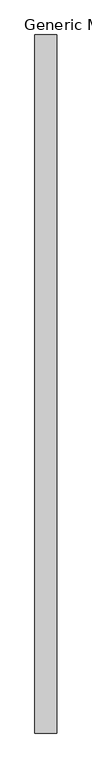
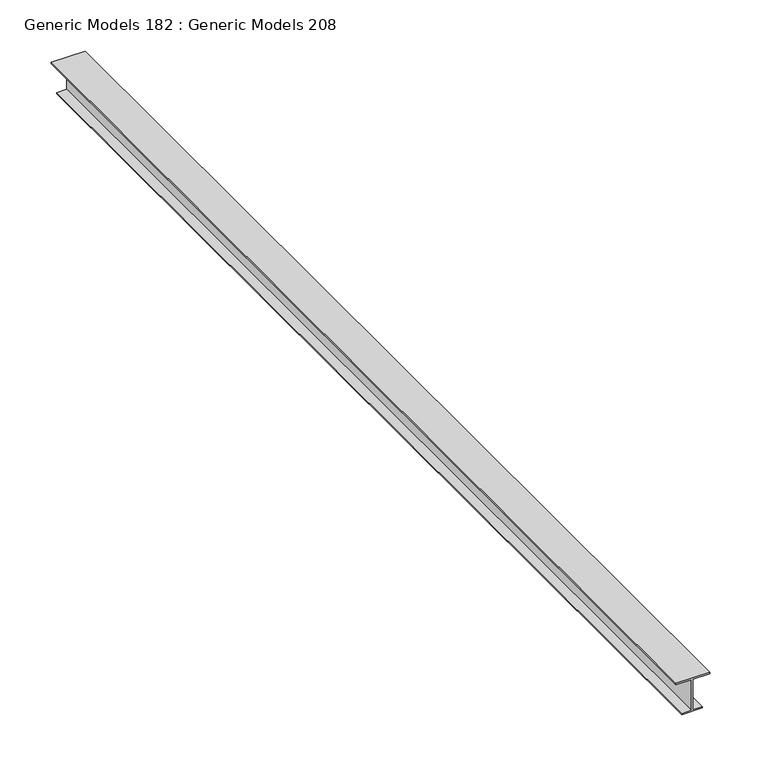
"""IFC4 building model written with IfcOpenShell, lengths in millimetres: proxy geometry, Generic Models 182 : Generic Models 208."""

from ifc_helpers import new_model, si_unit, frame, origin, place, context, project, spatial, polyline, outline, extrude, source, transform, mapped, element, save


def generic_models_182_generic_models_208_f42396d7(model_context):
    return source(origin(), model_context, "Body", "SweptSolid", [
        extrude(outline(polyline([(2185.2061106, 54757.0967998), (2183.6186106, 54757.0967998), (2183.6186106, 54774.5592998), (2147.1061106, 54774.5592998), (2147.1061106, 54763.537231), (2145.5186106, 54763.537231), (2145.5186106, 54787.1688685), (2147.1061106, 54787.1688685), (2147.1061106, 54776.1467998), (2183.6186106, 54776.1467998), (2183.6186106, 54795.1967998), (2185.2061106, 54795.1967998), (2185.2061106, 54757.0967998)])), frame((0.0, -228.7033818, 0.0), z_axis=(0.0, 1.0, 0.0), x_axis=(0.0, 0.0, 1.0)), (0.0, 0.0, 1.0), 1219.2),
    ])


if __name__ == "__main__":
    model = new_model("IFC4")
    model_context = context("Model", 3, world=origin())
    ifc_project = project(units=[si_unit("LENGTHUNIT", "METRE", prefix="MILLI")], contexts=[model_context])
    site = spatial("IfcSite", under=ifc_project)
    building = spatial("IfcBuilding", under=site)
    placement = place(None, origin())
    generic_models_182_generic_models_208_shape = generic_models_182_generic_models_208_f42396d7(model_context)
    element("IfcBuildingElementProxy", 1, Name="Generic Models 182 : Generic Models 208", ObjectType="Generic Models 182 : Generic Models 208", at=placement, inside=building, context=model_context, shape_type="MappedRepresentation", body=[
        mapped(generic_models_182_generic_models_208_shape, transform((0.0, 0.0, 0.0), x_axis=(1.0, 0.0, 0.0), y_axis=(0.0, 1.0, 0.0), z_axis=(0.0, 0.0, 1.0))),
    ])
    save(model, "model.ifc")
